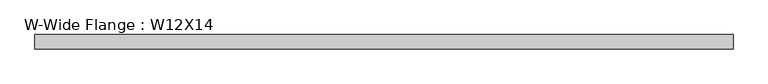
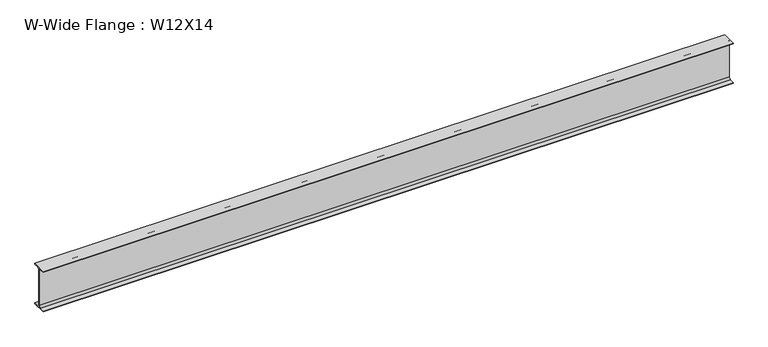
"""IFC4 building model written with IfcOpenShell, lengths in millimetres: beam geometry, W-Wide Flange : W12X14."""

from ifc_helpers import new_model, si_unit, point, frame, frame_2d, origin, place, context, project, spatial, polyline, circle_curve, trimmed, segment, composite_curve, outline, extrude, source, transform, mapped, element, save


def w_wide_flange_w12x14_7b406e19(model_context):
    return source(origin(), model_context, "Body", "SweptSolid", [
        extrude(outline(composite_curve([segment(polyline([(50.419, -145.415), (50.419, -151.13), (-50.419, -151.13), (-50.419, -145.415), (-15.875, -145.415)]), True, "CONTINUOUS"), segment(trimmed(circle_curve(frame_2d((-15.875, -132.08)), 13.335), [point((-15.875, -145.415))], [point((-2.54, -132.08))], True, "CARTESIAN"), True, "CONTINUOUS"), segment(polyline([(-2.54, -132.08), (-2.54, 132.08)]), True, "CONTINUOUS"), segment(trimmed(circle_curve(frame_2d((-15.875, 132.08)), 13.335), [point((-2.54, 132.08))], [point((-15.875, 145.415))], True, "CARTESIAN"), True, "CONTINUOUS"), segment(polyline([(-15.875, 145.415), (-50.419, 145.415), (-50.419, 151.13), (50.419, 151.13), (50.419, 145.415), (15.875, 145.415)]), True, "CONTINUOUS"), segment(trimmed(circle_curve(frame_2d((15.875, 132.08)), 13.335), [point((15.875, 145.415))], [point((2.54, 132.08))], True, "CARTESIAN"), True, "CONTINUOUS"), segment(polyline([(2.54, 132.08), (2.54, -132.08)]), True, "CONTINUOUS"), segment(trimmed(circle_curve(frame_2d((15.875, -132.08)), 13.335), [point((2.54, -132.08))], [point((15.875, -145.415))], True, "CARTESIAN"), True, "CONTINUOUS"), segment(polyline([(15.875, -145.415), (50.419, -145.415)]), True, "CONTINUOUS")], self_intersect=False)), frame((-2438.781, 0.0, 0.0), z_axis=(1.0, 0.0, 0.0), x_axis=(0.0, 1.0, 0.0)), (0.0, 0.0, 1.0), 4902.073),
    ])


if __name__ == "__main__":
    model = new_model("IFC4")
    model_context = context("Model", 3, world=origin())
    ifc_project = project(units=[si_unit("LENGTHUNIT", "METRE", prefix="MILLI")], contexts=[model_context])
    site = spatial("IfcSite", under=ifc_project)
    building = spatial("IfcBuilding", under=site)
    placement = place(None, origin())
    w_wide_flange_w12x14_shape = w_wide_flange_w12x14_7b406e19(model_context)
    element("IfcBeam", 1, ObjectType="W-Wide Flange : W12X14", at=placement, inside=building, context=model_context, shape_type="MappedRepresentation", body=[
        mapped(w_wide_flange_w12x14_shape, transform((0.0, 0.0, 0.0), x_axis=(1.0, 0.0, 0.0), y_axis=(0.0, 1.0, 0.0), z_axis=(0.0, 0.0, 1.0))),
    ])
    save(model, "model.ifc")

# Revit data of these elements
# Type "W-Wide Flange : W12X14"
#   Assembly Code = "B10"
#   W = 14
#   Length [instance default] = 5' - 0"
#   bf = 0' - 3.97"
#   d = 0' - 11.9"
#   k = 0' - 0 3/4"
#   k2 = 0' - 0.525"
#   tf = 0' - 0.225"
#   tw = 0' - 0.2"
#   A = 0.0288889 SF
#   Structural Material [instance default] = Steel ASTM A992
# Element 1 (IfcBeam, "W-Wide Flange : W12X14")
#   Materials on its faces: "Steel ASTM A992"
# Materials
#   "Steel ASTM A992": class "Metal", colour RGB 199 199 199, transparency 0, Description = "Structural steel 50ksi", Cost = 0
